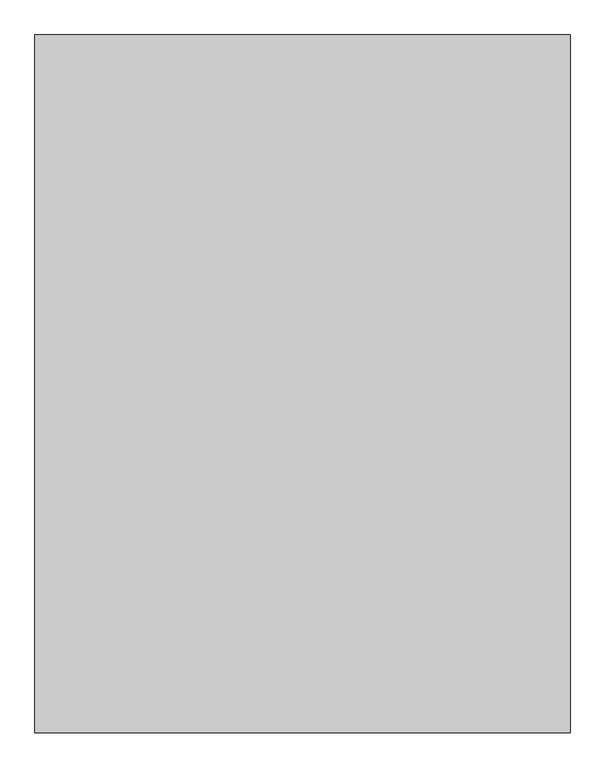
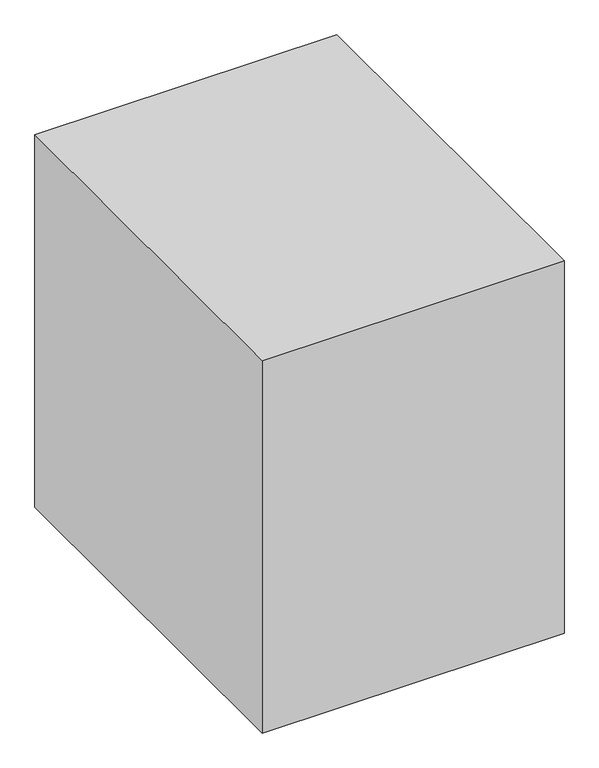
"""IFC4 building model written with IfcOpenShell, lengths in millimetres: proxy geometry, Space Planning Box_hec : Space Planning Box_hec."""

import ifcopenshell
import ifcopenshell.guid

model = None  # the IFC model being written
_history = None  # IfcOwnerHistory: only IFC2X3 demands one
_inside = {}  # id of a spatial element -> (the spatial element, [elements in it])
_under = {}  # id of a project, library or spatial element -> (it, [spatial elements below it])
_declared = {}  # id of a project -> (the project, [libraries it declares])
_typed = {}  # id of a type object -> (the type object, [elements of that type])
_made_of = {}  # id of a material, layer set ... -> (it, [elements and type objects made of it])


def new_model(schema):
    """Start an empty IFC model of exactly this schema.

    Asked for "IFC4X3", IfcOpenShell would pick the latest addendum, in which some entities
    have other attributes; the version numbers below select the first issue.
    IFC2X3 requires an IfcOwnerHistory on every rooted entity: one is made here for all.
    """
    global model, _history
    if schema == "IFC4X3":
        model = ifcopenshell.file(schema_version=(4, 3, 0, 0))
    else:
        model = ifcopenshell.file(schema=schema)
    _inside.clear()
    _under.clear()
    _declared.clear()
    _typed.clear()
    _made_of.clear()
    _history = None
    if model.schema == "IFC2X3":
        org = make("IfcOrganization", Name="unknown")
        user = make(
            "IfcPersonAndOrganization",
            ThePerson=make("IfcPerson", FamilyName="unknown"),
            TheOrganization=org,
        )
        app = make(
            "IfcApplication",
            ApplicationDeveloper=org,
            Version="unknown",
            ApplicationFullName="unknown",
            ApplicationIdentifier="unknown",
        )
        _history = make(
            "IfcOwnerHistory",
            OwningUser=user,
            OwningApplication=app,
            ChangeAction="ADDED",
            CreationDate=0,
        )
    return model


def make(cls, **values):
    """One entity of the class cls with the attributes given. An attribute that is None is left unset."""
    return model.create_entity(
        cls, **{name: value for name, value in values.items() if value is not None}
    )


def rooted(cls, **values):
    """An entity with a GlobalId (a new one), such as an element, a storey or a relation."""
    return make(cls, GlobalId=ifcopenshell.guid.new(), OwnerHistory=_history, **values)


def si_unit(unit_type, name, prefix=None):
    """IfcSIUnit, for example si_unit("LENGTHUNIT", "METRE", prefix="MILLI")."""
    return make("IfcSIUnit", UnitType=unit_type, Prefix=prefix, Name=name)


def assignment(units):
    """IfcUnitAssignment: the units of a project."""
    return None if units is None else make("IfcUnitAssignment", Units=units)


def point(xyz):
    """IfcCartesianPoint."""
    return None if xyz is None else make("IfcCartesianPoint", Coordinates=xyz)


def direction(xyz):
    """IfcDirection."""
    return None if xyz is None else make("IfcDirection", DirectionRatios=xyz)


def frame(location, z_axis=None, x_axis=None):
    """IfcAxis2Placement3D, a coordinate frame: its origin and axes. An axis left out is left unset."""
    return make(
        "IfcAxis2Placement3D",
        Location=point(location),
        Axis=direction(z_axis),
        RefDirection=direction(x_axis),
    )


def origin():
    """The frame at (0, 0, 0) with its axes left unset."""
    return frame((0.0, 0.0, 0.0))


def origin_with_axes():
    """The frame at (0, 0, 0) with the z axis (0, 0, 1) and the x axis (1, 0, 0) written out."""
    return frame((0.0, 0.0, 0.0), z_axis=(0.0, 0.0, 1.0), x_axis=(1.0, 0.0, 0.0))


def place(relative_to, where):
    """IfcLocalPlacement: puts the frame where relative to a parent placement (None: the world)."""
    return make(
        "IfcLocalPlacement", PlacementRelTo=relative_to, RelativePlacement=where
    )


def context(
    kind, dimensions, precision=None, world=None, true_north=None, identifier=None
):
    """IfcGeometricRepresentationContext, for example the 3D "Model" context."""
    return make(
        "IfcGeometricRepresentationContext",
        ContextIdentifier=identifier,
        ContextType=kind,
        CoordinateSpaceDimension=dimensions,
        Precision=precision,
        WorldCoordinateSystem=world,
        TrueNorth=true_north,
    )


def project(units=None, contexts=None):
    """IfcProject with its units and contexts."""
    return rooted(
        "IfcProject",
        Name="project",
        RepresentationContexts=contexts,
        UnitsInContext=assignment(units),
    )


def spatial(cls, under=None, at=None, **own):
    """A site, building, storey or space (cls), placed at a placement, below another one or the project."""
    s = rooted(cls, ObjectPlacement=at, **own)
    if under is not None:
        _under.setdefault(under.id(), (under, []))[1].append(s)
    return s


def polyline(points):
    """IfcPolyline through the points."""
    return make("IfcPolyline", Points=[point(p) for p in points])


def outline(outer, holes=None, kind="AREA"):
    """IfcArbitraryClosedProfileDef: a profile drawn as a closed curve; with holes, ...WithVoids."""
    if holes is None:
        return make("IfcArbitraryClosedProfileDef", ProfileType=kind, OuterCurve=outer)
    return make(
        "IfcArbitraryProfileDefWithVoids",
        ProfileType=kind,
        OuterCurve=outer,
        InnerCurves=holes,
    )


def extrude(swept, where, along, depth):
    """IfcExtrudedAreaSolid: the profile swept, set in the frame where, extruded along a direction by depth."""
    return make(
        "IfcExtrudedAreaSolid",
        SweptArea=swept,
        Position=where,
        ExtrudedDirection=direction(along),
        Depth=depth,
    )


def shape(context_of_items, identifier, shape_type, items):
    """IfcShapeRepresentation: the items that make up one representation, for example the "Body"."""
    return make(
        "IfcShapeRepresentation",
        ContextOfItems=context_of_items,
        RepresentationIdentifier=identifier,
        RepresentationType=shape_type,
        Items=items,
    )


def source(mapping_origin, context_of_items, identifier, shape_type, items):
    """IfcRepresentationMap: a shape defined once, which mapped items show again and again."""
    return make(
        "IfcRepresentationMap",
        MappingOrigin=mapping_origin,
        MappedRepresentation=shape(context_of_items, identifier, shape_type, items),
    )


def transform(
    local_origin,
    x_axis=None,
    y_axis=None,
    z_axis=None,
    scale=None,
    scale2=None,
    scale3=None,
    uniform=True,
):
    """IfcCartesianTransformationOperator3D, or its non-uniform kind. x_axis, y_axis, z_axis: its Axis1, 2, 3."""
    if uniform:
        return make(
            "IfcCartesianTransformationOperator3D",
            Axis1=direction(x_axis),
            Axis2=direction(y_axis),
            LocalOrigin=point(local_origin),
            Scale=scale,
            Axis3=direction(z_axis),
        )
    return make(
        "IfcCartesianTransformationOperator3DnonUniform",
        Axis1=direction(x_axis),
        Axis2=direction(y_axis),
        LocalOrigin=point(local_origin),
        Scale=scale,
        Axis3=direction(z_axis),
        Scale2=scale2,
        Scale3=scale3,
    )


def mapped(mapping_source, mapping_target):
    """IfcMappedItem: shows the shape of a source again, moved by a transform."""
    return make(
        "IfcMappedItem", MappingSource=mapping_source, MappingTarget=mapping_target
    )


def made_of(thing, what):
    """Note that an element or type object is made of a material, layer set ...; save() writes the relation."""
    if what is not None:
        _made_of.setdefault(what.id(), (what, []))[1].append(thing)
    return thing


def element(
    cls,
    number,
    at=None,
    inside=None,
    cuts=None,
    type_object=None,
    material=None,
    context=None,
    identifier="Body",
    shape_type=None,
    held_by="IfcProductDefinitionShape",
    body=None,
    shapes=None,
    **own,
):
    """One element of the class cls, such as IfcWall. Its Tag is "e" and its number.

    at: its placement. inside: the storey or other place that contains it. cuts: it is an
    opening in that element (IfcRelVoidsElement). A single representation is given by context,
    identifier, shape_type and body (its items); several are given by shapes. held_by: the class
    of the entity that holds the representations. save() writes the other relations.
    """
    e = rooted(cls, Tag="e%d" % number, ObjectPlacement=at, **own)
    if body is not None:
        shapes = [shape(context, identifier, shape_type, body)]
    if shapes is not None:
        e.Representation = make(held_by, Representations=shapes)
    if inside is not None:
        _inside.setdefault(inside.id(), (inside, []))[1].append(e)
    if cuts is not None:
        rooted(
            "IfcRelVoidsElement", RelatingBuildingElement=cuts, RelatedOpeningElement=e
        )
    if type_object is not None:
        _typed.setdefault(type_object.id(), (type_object, []))[1].append(e)
    return made_of(e, material)


def aggregate(whole, parts):
    """IfcRelAggregates: a whole, such as a stair, and the parts it consists of."""
    return rooted("IfcRelAggregates", RelatingObject=whole, RelatedObjects=parts)


def save(model, path):
    """Write the relations noted so far, then the file.

    IfcRelAggregates (storeys below a building ...), IfcRelContainedInSpatialStructure (elements
    in a storey), IfcRelDefinesByType, IfcRelAssociatesMaterial and IfcRelDeclares: one each for
    every whole, place, type object, material and project.
    """
    for whole, parts in _under.values():
        aggregate(whole, parts)
    for where, things in _inside.values():
        rooted(
            "IfcRelContainedInSpatialStructure",
            RelatedElements=things,
            RelatingStructure=where,
        )
    for kind, things in _typed.values():
        rooted("IfcRelDefinesByType", RelatedObjects=things, RelatingType=kind)
    for what, things in _made_of.values():
        rooted("IfcRelAssociatesMaterial", RelatedObjects=things, RelatingMaterial=what)
    for by, libraries in _declared.values():
        rooted("IfcRelDeclares", RelatingContext=by, RelatedDefinitions=libraries)
    model.write(path)


def generic_models_1a87c0f4(model_context):
    return source(origin(), model_context, "Body", "SweptSolid", [
        extrude(outline(polyline([(2300.0, 3000.0), (2300.0, -3000.0), (-2300.0, -3000.0), (-2300.0, 3000.0), (2300.0, 3000.0)])), origin_with_axes(), (0.0, 0.0, 1.0), 6000.0),
    ])


if __name__ == "__main__":
    model = new_model("IFC4")
    model_context = context("Model", 3, world=origin())
    ifc_project = project(units=[si_unit("LENGTHUNIT", "METRE", prefix="MILLI")], contexts=[model_context])
    site = spatial("IfcSite", under=ifc_project)
    building = spatial("IfcBuilding", under=site)
    placement = place(None, origin())
    generic_models_shape = generic_models_1a87c0f4(model_context)
    element("IfcBuildingElementProxy", 1, Name="Space Planning Box_hec : Space Planning Box_hec", ObjectType="Space Planning Box_hec : Space Planning Box_hec", at=placement, inside=building, context=model_context, shape_type="MappedRepresentation", body=[
        mapped(generic_models_shape, transform((0.0, 0.0, 0.0), x_axis=(1.0, 0.0, 0.0), y_axis=(0.0, 1.0, 0.0), z_axis=(0.0, 0.0, 1.0))),
    ])
    save(model, "model.ifc")

# Revit data of these elements
# Project information
#   Building Name = "MAIN GATE SECURITY BUILDING"
#   Project Status = "Project Status"
#   Client Name = "현대엔지니어링"
#   Project Address = "서울시 종로구 율곡로 75(계동)"
#   Project Name = "Therma Visayas Energy Project"
#   Project Number = "-"
# Type "Space Planning Box_hec : Space Planning Box_hec"
#   Type Comments = "..."
#   Room Name [instance default] = "?"
#   Interior Finish [instance default] = ""
#   Exterior Finish [instance default] = ""
#   Department [instance default] = ""
#   Assembly Code = "..."
#   Width [instance default] = 1524 mm
#   Program Area [instance default] = 0.00 m²
#   Length [instance default] = 1524 mm
#   Height [instance default] = 1524 mm
#   Area [instance default] = 2.32258 m²
#   Fill Color [instance default] = Cyan
#   Default Elevation = 0
# Element 1 (IfcBuildingElementProxy, "Space Planning Box_hec : Space Planning Box_hec")
#   Room Name = "Document Room"
#   Interior Finish = "IF2-1"
#   Exterior Finish = "EF1"
#   Department = "AR"
#   Width = 4600 mm
#   Program Area = 48.00 m²
#   Length = 6000 mm
#   Height = 6000 mm
#   Area = 27.60 m²
#   Fill Color = Lavender
#   Materials on its faces: "Lavender"
# Materials
#   "Cyan": class "Generic", colour RGB 0 255 255, transparency 0.2, Cost = 0
#   "Lavender": class "Generic", colour RGB 186 85 211, transparency 0.2, Cost = 0
